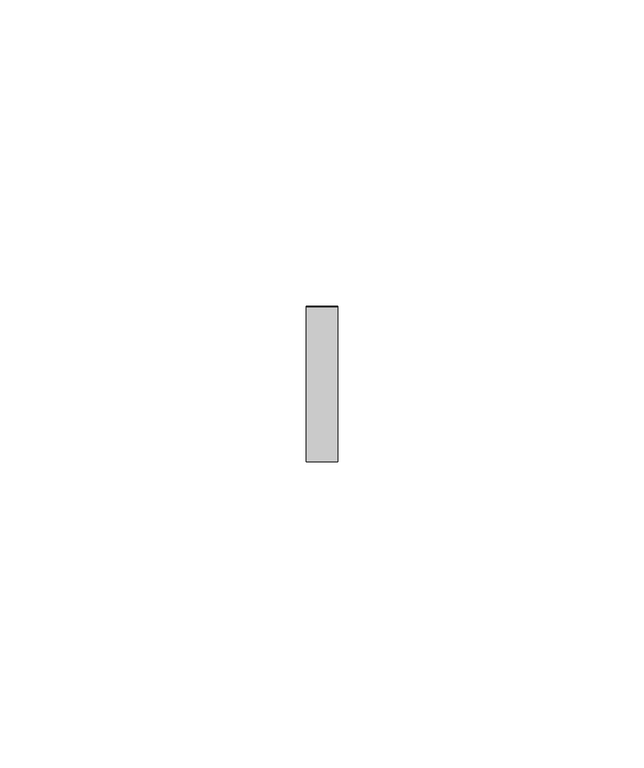
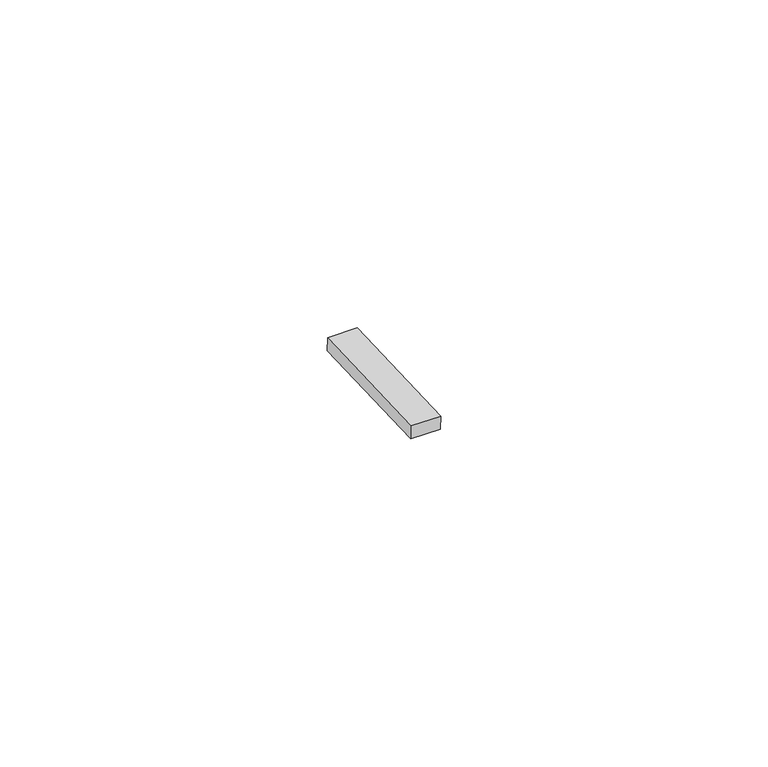
"""IFC4 building model written with IfcOpenShell, lengths in millimetres: proxy geometry, Inner panel:Inner panel:1:Inner panel:1 : Inner panel:Inner panel:300324:2:Inner panel:1:Inner panel:1 : Inner panel:Inner panel:300324:2 : Inner panel:Inner panel:1:Inner panel:1 : Inner panel:Inner panel:300324:300043:119 : Inner panel:Inner panel:1:Inner panel:1 : Inner panel:Inner panel:300324:2:Inner panel:1:Inner panel:1 : Inner panel:Inner panel:300324:2 : Inner panel:Inner panel:1:Inner panel:1 : Inner panel:Inner panel:300324:300043:308120."""

import ifcopenshell
import ifcopenshell.guid

model = None  # the IFC model being written
_history = None  # IfcOwnerHistory: only IFC2X3 demands one
_inside = {}  # id of a spatial element -> (the spatial element, [elements in it])
_under = {}  # id of a project, library or spatial element -> (it, [spatial elements below it])
_declared = {}  # id of a project -> (the project, [libraries it declares])
_typed = {}  # id of a type object -> (the type object, [elements of that type])
_made_of = {}  # id of a material, layer set ... -> (it, [elements and type objects made of it])


def new_model(schema):
    """Start an empty IFC model of exactly this schema.

    Asked for "IFC4X3", IfcOpenShell would pick the latest addendum, in which some entities
    have other attributes; the version numbers below select the first issue.
    IFC2X3 requires an IfcOwnerHistory on every rooted entity: one is made here for all.
    """
    global model, _history
    if schema == "IFC4X3":
        model = ifcopenshell.file(schema_version=(4, 3, 0, 0))
    else:
        model = ifcopenshell.file(schema=schema)
    _inside.clear()
    _under.clear()
    _declared.clear()
    _typed.clear()
    _made_of.clear()
    _history = None
    if model.schema == "IFC2X3":
        org = make("IfcOrganization", Name="unknown")
        user = make(
            "IfcPersonAndOrganization",
            ThePerson=make("IfcPerson", FamilyName="unknown"),
            TheOrganization=org,
        )
        app = make(
            "IfcApplication",
            ApplicationDeveloper=org,
            Version="unknown",
            ApplicationFullName="unknown",
            ApplicationIdentifier="unknown",
        )
        _history = make(
            "IfcOwnerHistory",
            OwningUser=user,
            OwningApplication=app,
            ChangeAction="ADDED",
            CreationDate=0,
        )
    return model


def make(cls, **values):
    """One entity of the class cls with the attributes given. An attribute that is None is left unset."""
    return model.create_entity(
        cls, **{name: value for name, value in values.items() if value is not None}
    )


def rooted(cls, **values):
    """An entity with a GlobalId (a new one), such as an element, a storey or a relation."""
    return make(cls, GlobalId=ifcopenshell.guid.new(), OwnerHistory=_history, **values)


def si_unit(unit_type, name, prefix=None):
    """IfcSIUnit, for example si_unit("LENGTHUNIT", "METRE", prefix="MILLI")."""
    return make("IfcSIUnit", UnitType=unit_type, Prefix=prefix, Name=name)


def assignment(units):
    """IfcUnitAssignment: the units of a project."""
    return None if units is None else make("IfcUnitAssignment", Units=units)


def point(xyz):
    """IfcCartesianPoint."""
    return None if xyz is None else make("IfcCartesianPoint", Coordinates=xyz)


def direction(xyz):
    """IfcDirection."""
    return None if xyz is None else make("IfcDirection", DirectionRatios=xyz)


def frame(location, z_axis=None, x_axis=None):
    """IfcAxis2Placement3D, a coordinate frame: its origin and axes. An axis left out is left unset."""
    return make(
        "IfcAxis2Placement3D",
        Location=point(location),
        Axis=direction(z_axis),
        RefDirection=direction(x_axis),
    )


def origin():
    """The frame at (0, 0, 0) with its axes left unset."""
    return frame((0.0, 0.0, 0.0))


def place(relative_to, where):
    """IfcLocalPlacement: puts the frame where relative to a parent placement (None: the world)."""
    return make(
        "IfcLocalPlacement", PlacementRelTo=relative_to, RelativePlacement=where
    )


def context(
    kind, dimensions, precision=None, world=None, true_north=None, identifier=None
):
    """IfcGeometricRepresentationContext, for example the 3D "Model" context."""
    return make(
        "IfcGeometricRepresentationContext",
        ContextIdentifier=identifier,
        ContextType=kind,
        CoordinateSpaceDimension=dimensions,
        Precision=precision,
        WorldCoordinateSystem=world,
        TrueNorth=true_north,
    )


def project(units=None, contexts=None):
    """IfcProject with its units and contexts."""
    return rooted(
        "IfcProject",
        Name="project",
        RepresentationContexts=contexts,
        UnitsInContext=assignment(units),
    )


def spatial(cls, under=None, at=None, **own):
    """A site, building, storey or space (cls), placed at a placement, below another one or the project."""
    s = rooted(cls, ObjectPlacement=at, **own)
    if under is not None:
        _under.setdefault(under.id(), (under, []))[1].append(s)
    return s


def polyline(points):
    """IfcPolyline through the points."""
    return make("IfcPolyline", Points=[point(p) for p in points])


def outline(outer, holes=None, kind="AREA"):
    """IfcArbitraryClosedProfileDef: a profile drawn as a closed curve; with holes, ...WithVoids."""
    if holes is None:
        return make("IfcArbitraryClosedProfileDef", ProfileType=kind, OuterCurve=outer)
    return make(
        "IfcArbitraryProfileDefWithVoids",
        ProfileType=kind,
        OuterCurve=outer,
        InnerCurves=holes,
    )


def extrude(swept, where, along, depth):
    """IfcExtrudedAreaSolid: the profile swept, set in the frame where, extruded along a direction by depth."""
    return make(
        "IfcExtrudedAreaSolid",
        SweptArea=swept,
        Position=where,
        ExtrudedDirection=direction(along),
        Depth=depth,
    )


def shape(context_of_items, identifier, shape_type, items):
    """IfcShapeRepresentation: the items that make up one representation, for example the "Body"."""
    return make(
        "IfcShapeRepresentation",
        ContextOfItems=context_of_items,
        RepresentationIdentifier=identifier,
        RepresentationType=shape_type,
        Items=items,
    )


def source(mapping_origin, context_of_items, identifier, shape_type, items):
    """IfcRepresentationMap: a shape defined once, which mapped items show again and again."""
    return make(
        "IfcRepresentationMap",
        MappingOrigin=mapping_origin,
        MappedRepresentation=shape(context_of_items, identifier, shape_type, items),
    )


def transform(
    local_origin,
    x_axis=None,
    y_axis=None,
    z_axis=None,
    scale=None,
    scale2=None,
    scale3=None,
    uniform=True,
):
    """IfcCartesianTransformationOperator3D, or its non-uniform kind. x_axis, y_axis, z_axis: its Axis1, 2, 3."""
    if uniform:
        return make(
            "IfcCartesianTransformationOperator3D",
            Axis1=direction(x_axis),
            Axis2=direction(y_axis),
            LocalOrigin=point(local_origin),
            Scale=scale,
            Axis3=direction(z_axis),
        )
    return make(
        "IfcCartesianTransformationOperator3DnonUniform",
        Axis1=direction(x_axis),
        Axis2=direction(y_axis),
        LocalOrigin=point(local_origin),
        Scale=scale,
        Axis3=direction(z_axis),
        Scale2=scale2,
        Scale3=scale3,
    )


def mapped(mapping_source, mapping_target):
    """IfcMappedItem: shows the shape of a source again, moved by a transform."""
    return make(
        "IfcMappedItem", MappingSource=mapping_source, MappingTarget=mapping_target
    )


def made_of(thing, what):
    """Note that an element or type object is made of a material, layer set ...; save() writes the relation."""
    if what is not None:
        _made_of.setdefault(what.id(), (what, []))[1].append(thing)
    return thing


def element(
    cls,
    number,
    at=None,
    inside=None,
    cuts=None,
    type_object=None,
    material=None,
    context=None,
    identifier="Body",
    shape_type=None,
    held_by="IfcProductDefinitionShape",
    body=None,
    shapes=None,
    **own,
):
    """One element of the class cls, such as IfcWall. Its Tag is "e" and its number.

    at: its placement. inside: the storey or other place that contains it. cuts: it is an
    opening in that element (IfcRelVoidsElement). A single representation is given by context,
    identifier, shape_type and body (its items); several are given by shapes. held_by: the class
    of the entity that holds the representations. save() writes the other relations.
    """
    e = rooted(cls, Tag="e%d" % number, ObjectPlacement=at, **own)
    if body is not None:
        shapes = [shape(context, identifier, shape_type, body)]
    if shapes is not None:
        e.Representation = make(held_by, Representations=shapes)
    if inside is not None:
        _inside.setdefault(inside.id(), (inside, []))[1].append(e)
    if cuts is not None:
        rooted(
            "IfcRelVoidsElement", RelatingBuildingElement=cuts, RelatedOpeningElement=e
        )
    if type_object is not None:
        _typed.setdefault(type_object.id(), (type_object, []))[1].append(e)
    return made_of(e, material)


def aggregate(whole, parts):
    """IfcRelAggregates: a whole, such as a stair, and the parts it consists of."""
    return rooted("IfcRelAggregates", RelatingObject=whole, RelatedObjects=parts)


def save(model, path):
    """Write the relations noted so far, then the file.

    IfcRelAggregates (storeys below a building ...), IfcRelContainedInSpatialStructure (elements
    in a storey), IfcRelDefinesByType, IfcRelAssociatesMaterial and IfcRelDeclares: one each for
    every whole, place, type object, material and project.
    """
    for whole, parts in _under.values():
        aggregate(whole, parts)
    for where, things in _inside.values():
        rooted(
            "IfcRelContainedInSpatialStructure",
            RelatedElements=things,
            RelatingStructure=where,
        )
    for kind, things in _typed.values():
        rooted("IfcRelDefinesByType", RelatedObjects=things, RelatingType=kind)
    for what, things in _made_of.values():
        rooted("IfcRelAssociatesMaterial", RelatedObjects=things, RelatingMaterial=what)
    for by, libraries in _declared.values():
        rooted("IfcRelDeclares", RelatingContext=by, RelatedDefinitions=libraries)
    model.write(path)


def generic_models_5dc7b884(model_context):
    return source(origin(), model_context, "Body", "SweptSolid", [
        extrude(outline(polyline([(0.0, -25.3999999), (0.0, 0.0), (5.2138089, 0.0), (5.2138089, -25.3999999), (0.0, -25.3999999)])), frame((592717.395117, -578962.7476805, 3951.4793391), z_axis=(0.0, -0.041630544712223896, 0.9991330730923502), x_axis=(-1.0, 0.0, 0.0)), (0.0, 0.0, 1.0), 2.4763745),
    ])


if __name__ == "__main__":
    model = new_model("IFC4")
    model_context = context("Model", 3, world=origin())
    ifc_project = project(units=[si_unit("LENGTHUNIT", "METRE", prefix="MILLI")], contexts=[model_context])
    site = spatial("IfcSite", under=ifc_project)
    building = spatial("IfcBuilding", under=site)
    placement = place(None, origin())
    generic_models_shape = generic_models_5dc7b884(model_context)
    element("IfcBuildingElementProxy", 1, Name="Inner panel:Inner panel:1:Inner panel:1 : Inner panel:Inner panel:300324:2:Inner panel:1:Inner panel:1 : Inner panel:Inner panel:300324:2 : Inner panel:Inner panel:1:Inner panel:1 : Inner panel:Inner panel:300324:300043:119 : Inner panel:Inner panel:1:Inner panel:1 : Inner panel:Inner panel:300324:2:Inner panel:1:Inner panel:1 : Inner panel:Inner panel:300324:2 : Inner panel:Inner panel:1:Inner panel:1 : Inner panel:Inner panel:300324:300043:308120", ObjectType="Inner panel:Inner panel:1:Inner panel:1 : Inner panel:Inner panel:300324:2:Inner panel:1:Inner panel:1 : Inner panel:Inner panel:300324:2 : Inner panel:Inner panel:1:Inner panel:1 : Inner panel:Inner panel:300324:300043:119 : Inner panel:Inner panel:1:Inner panel:1 : Inner panel:Inner panel:300324:2:Inner panel:1:Inner panel:1 : Inner panel:Inner panel:300324:2 : Inner panel:Inner panel:1:Inner panel:1 : Inner panel:Inner panel:300324:300043:308120", at=placement, inside=building, context=model_context, shape_type="MappedRepresentation", body=[
        mapped(generic_models_shape, transform((0.0, 0.0, 0.0), x_axis=(1.0, 0.0, 0.0), y_axis=(0.0, 1.0, 0.0), z_axis=(0.0, 0.0, 1.0))),
    ])
    save(model, "model.ifc")

# Revit data of these elements
# Type "Inner panel:Inner panel:1:Inner panel:1 : Inner panel:Inner panel:300324:2:Inner panel:1:Inner panel:1 : Inner panel:Inner panel:300324:2 : Inner panel:Inner panel:1:Inner panel:1 : Inner panel:Inner panel:300324:300043:119 : Inner panel:Inner panel:1:Inner panel:1 : Inner panel:Inner panel:300324:2:Inner panel:1:Inner panel:1 : Inner panel:Inner panel:300324:2 : Inner panel:Inner panel:1:Inner panel:1 : Inner panel:Inner panel:300324:300043:308120"
#   NameOverride = "Inner panel:Inner panel:1:Inner panel:1 : Inner panel:Inner panel:300324:2:Inner panel:1:Inner panel:1 : Inner panel:Inner panel:300324:2 : Inner panel:Inner panel:1:Inner panel:1 : Inner panel:Inner panel:300324:300043:308120"
#   ObjectTypeOverride = "Inner panel:1:Inner panel:1 : Inner panel:Inner panel:300324:2 : Inner panel:Inner panel:1:Inner panel:1 : Inner panel:Inner panel:300324:300043"
#   Reference = "Inner panel"
#   Tag = "308120"
# Element 1 (IfcBuildingElementProxy, "Inner panel:Inner panel:1:Inner panel:1 : Inner panel:Inner panel:300324:2:Inner panel:1:Inner panel:1 : Inner panel:Inner panel:300324:2 : Inner panel:Inner panel:1:Inner panel:1 : Inner panel:Inner panel:300324:300043:119 : Inner panel:Inner panel:1:Inner panel:1 : Inner panel:Inner panel:300324:2:Inner panel:1:Inner panel:1 : Inner panel:Inner panel:300324:2 : Inner panel:Inner panel:1:Inner panel:1 : Inner panel:Inner panel:300324:300043:308120")
#   Materials on its faces: "AT CLIP - 1\" WIDE NON ABSORBENT, WEATHER-RESISTANT NEOPRENE/EPDM/SBR FOAM"
# Materials
#   "AT CLIP - 1\" WIDE NON ABSORBENT, WEATHER-RESISTANT NEOPRENE/EPDM/SBR FOAM": class "Generic", colour RGB 85 85 85, transparency 0, Cost = 0
